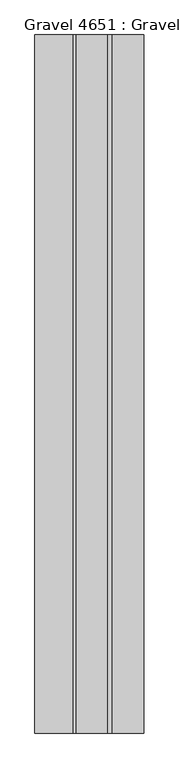
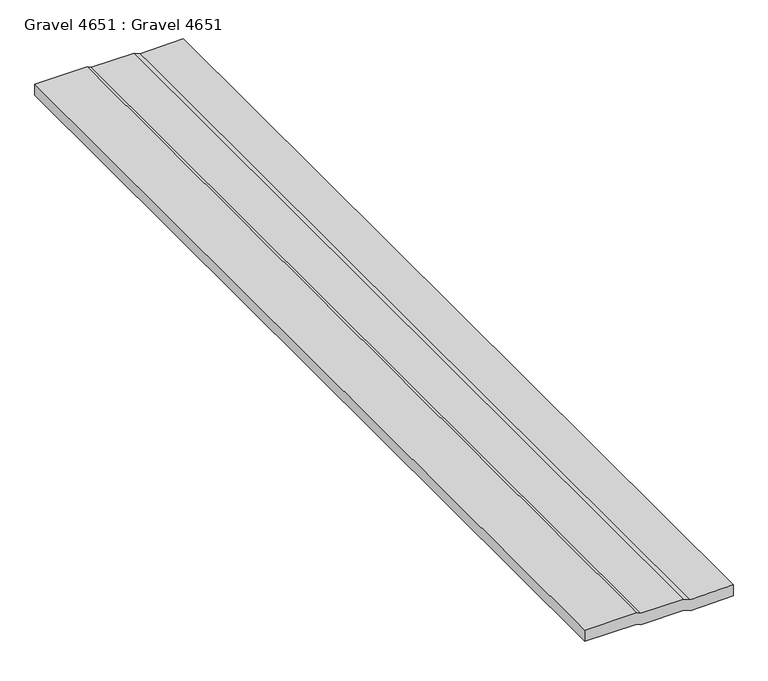
"""IFC4 building model written with IfcOpenShell, lengths in millimetres: proxy geometry, Gravel 4651 : Gravel 4651."""

from ifc_helpers import new_model, si_unit, frame, origin, place, context, project, spatial, polyline, outline, extrude, source, transform, mapped, element, save


def gravel_4651_gravel_4651_052f081c(model_context):
    return source(origin(), model_context, "Body", "SweptSolid", [
        extrude(outline(polyline([(40274.2359464, -4902.3767758), (40269.9546964, -4893.6663265), (40269.9546964, -4803.0794125), (40264.2272344, -4790.2347731), (40265.8726651, -4699.8063764), (40290.6109464, -4699.8063764), (40288.9655157, -4790.2347731), (40294.6929777, -4803.0794125), (40294.6929777, -4893.6663265), (40298.9742277, -4902.3767758), (40298.9742277, -5011.8762875), (40274.2359464, -5011.8762875), (40274.2359464, -4902.3767758)])), frame((0.0, -1052.6406573, 0.0), z_axis=(0.0, 1.0, 0.0), x_axis=(0.0, 0.0, 1.0)), (0.0, 0.0, 1.0), 2000.0),
    ])


if __name__ == "__main__":
    model = new_model("IFC4")
    model_context = context("Model", 3, world=origin())
    ifc_project = project(units=[si_unit("LENGTHUNIT", "METRE", prefix="MILLI")], contexts=[model_context])
    site = spatial("IfcSite", under=ifc_project)
    building = spatial("IfcBuilding", under=site)
    placement = place(None, origin())
    gravel_4651_gravel_4651_shape = gravel_4651_gravel_4651_052f081c(model_context)
    element("IfcBuildingElementProxy", 1, Name="Gravel 4651 : Gravel 4651", ObjectType="Gravel 4651 : Gravel 4651", at=placement, inside=building, context=model_context, shape_type="MappedRepresentation", body=[
        mapped(gravel_4651_gravel_4651_shape, transform((0.0, 0.0, 0.0), x_axis=(1.0, 0.0, 0.0), y_axis=(0.0, 1.0, 0.0), z_axis=(0.0, 0.0, 1.0))),
    ])
    save(model, "model.ifc")

# Revit data of these elements
# Type "Gravel 4651 : Gravel 4651"
#   NameOverride = "Gravel"
# Element 1 (IfcBuildingElementProxy, "Gravel 4651 : Gravel 4651")
#   Materials on its faces: "GRAVEL BALLAST"
# Materials
#   "GRAVEL BALLAST": class "Unassigned", colour RGB 128 128 128, transparency 0, Cost = 0
